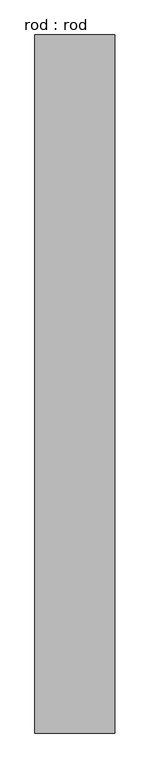
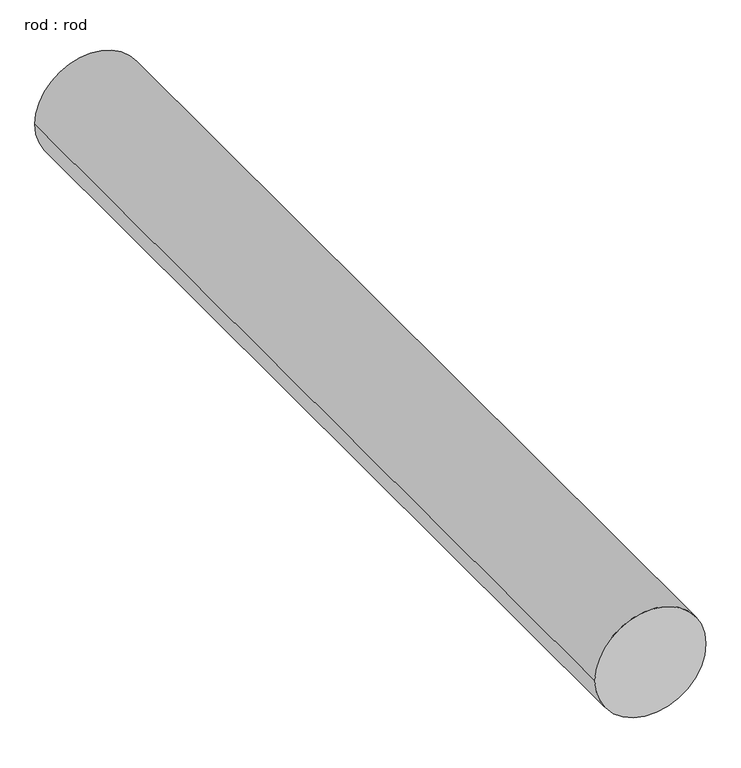
"""IFC4 building model written with IfcOpenShell, lengths in millimetres: proxy geometry, rod : rod."""

from ifc_helpers import new_model, si_unit, point, frame, frame_2d, origin, place, context, project, spatial, circle_curve, trimmed, segment, composite_curve, outline, extrude, source, transform, mapped, element, save


def rod_rod_2703f145(model_context):
    return source(origin(), model_context, "Body", "SweptSolid", [
        extrude(outline(composite_curve([segment(trimmed(circle_curve(frame_2d((0.0108462, 0.0)), 200.0), [point((0.0108462, 200.0))], [point((0.0108462, -200.0))], False, "CARTESIAN"), True, "CONTINUOUS"), segment(trimmed(circle_curve(frame_2d((0.0108462, 0.0)), 200.0), [point((0.0108462, -200.0))], [point((0.0108462, 200.0))], False, "CARTESIAN"), True, "CONTINUOUS")], self_intersect=False)), frame((0.0, 2346.3000439, 0.0), z_axis=(0.0, 1.0, 0.0), x_axis=(0.0, 0.0, 1.0)), (0.0, 0.0, 1.0), 3492.8571429),
    ])


if __name__ == "__main__":
    model = new_model("IFC4")
    model_context = context("Model", 3, world=origin())
    ifc_project = project(units=[si_unit("LENGTHUNIT", "METRE", prefix="MILLI")], contexts=[model_context])
    site = spatial("IfcSite", under=ifc_project)
    building = spatial("IfcBuilding", under=site)
    placement = place(None, origin())
    rod_rod_shape = rod_rod_2703f145(model_context)
    element("IfcBuildingElementProxy", 1, Name="rod : rod", ObjectType="rod : rod", at=placement, inside=building, context=model_context, shape_type="MappedRepresentation", body=[
        mapped(rod_rod_shape, transform((0.0, 0.0, 0.0), x_axis=(1.0, 0.0, 0.0), y_axis=(0.0, 1.0, 0.0), z_axis=(0.0, 0.0, 1.0))),
    ])
    save(model, "model.ifc")

# Revit data of these elements
# Type "rod : rod"
#   Default Elevation = 0
